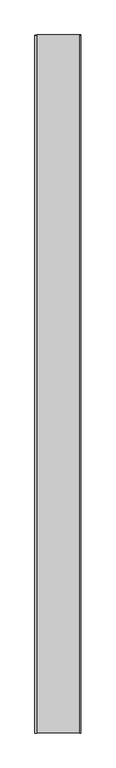
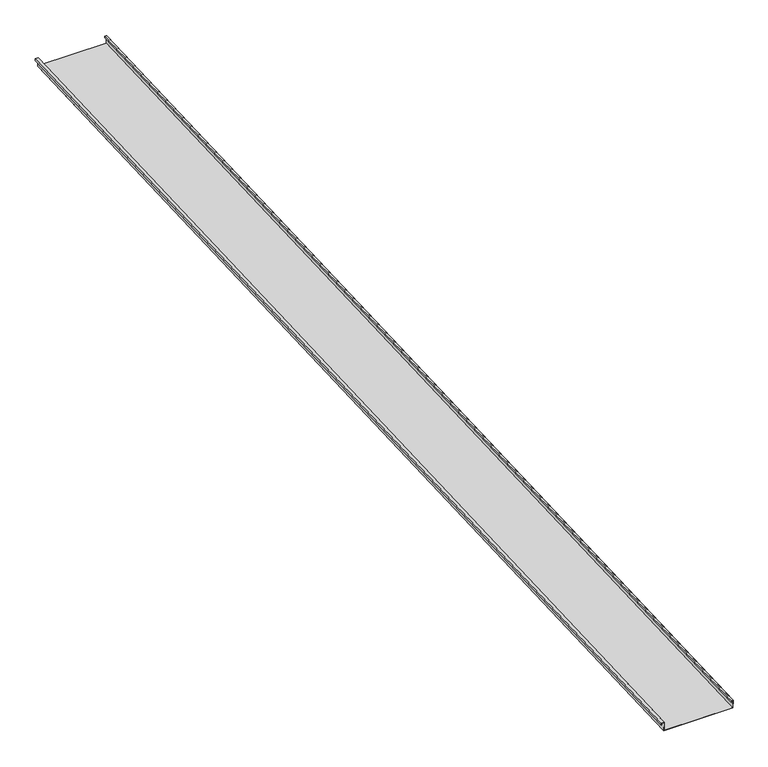
"""IFC4 building model written with IfcOpenShell, lengths in millimetres: proxy geometry, Generic Models 2:Generic Models 2:310765:Generic Models 2:310765 : Generic Models 2:Generic Models 2:310765:112 : Generic Models 2:Generic Models 2:310765:Generic Models 2:310765 : Generic Models 2:Generic Models 2:310765:300385."""

from ifc_helpers import new_model, si_unit, frame, origin, place, context, project, spatial, polyline, outline, extrude, source, transform, mapped, element, save


def generic_models_0e6c4cea(model_context):
    return source(origin(), model_context, "Body", "SweptSolid", [
        extrude(outline(polyline([(1.5875, 0.0), (1.5875, 50.8), (407.9875, 50.8), (407.9875, 1.5875), (396.875, 1.5875), (396.875, 11.1125), (398.4625, 11.1125), (398.4625, 3.175), (406.4, 3.175), (406.4, 49.2125), (3.175, 49.2125), (3.175, -1.5874999), (-14.2875, -1.5874999), (-14.2875, 9.525), (-12.7, 9.525), (-12.7, 0.0), (1.5875, 0.0)])), frame((608242.8096406, -581354.4345603, 3902.6697972), z_axis=(0.0, 0.9991330730923568, 0.041630544712067834), x_axis=(1.0, 0.0, 0.0)), (0.0, 0.0, 1.0), 6400.8),
    ])


if __name__ == "__main__":
    model = new_model("IFC4")
    model_context = context("Model", 3, world=origin())
    ifc_project = project(units=[si_unit("LENGTHUNIT", "METRE", prefix="MILLI")], contexts=[model_context])
    site = spatial("IfcSite", under=ifc_project)
    building = spatial("IfcBuilding", under=site)
    placement = place(None, origin())
    generic_models_shape = generic_models_0e6c4cea(model_context)
    element("IfcBuildingElementProxy", 1, Name="Generic Models 2:Generic Models 2:310765:Generic Models 2:310765 : Generic Models 2:Generic Models 2:310765:112 : Generic Models 2:Generic Models 2:310765:Generic Models 2:310765 : Generic Models 2:Generic Models 2:310765:300385", ObjectType="Generic Models 2:Generic Models 2:310765:Generic Models 2:310765 : Generic Models 2:Generic Models 2:310765:112 : Generic Models 2:Generic Models 2:310765:Generic Models 2:310765 : Generic Models 2:Generic Models 2:310765:300385", at=placement, inside=building, context=model_context, shape_type="MappedRepresentation", body=[
        mapped(generic_models_shape, transform((0.0, 0.0, 0.0), x_axis=(1.0, 0.0, 0.0), y_axis=(0.0, 1.0, 0.0), z_axis=(0.0, 0.0, 1.0))),
    ])
    save(model, "model.ifc")

# Revit data of these elements
# Type "Generic Models 2:Generic Models 2:310765:Generic Models 2:310765 : Generic Models 2:Generic Models 2:310765:112 : Generic Models 2:Generic Models 2:310765:Generic Models 2:310765 : Generic Models 2:Generic Models 2:310765:300385"
#   NameOverride = "Generic Models 2:Generic Models 2:310765:Generic Models 2:310765 : Generic Models 2:Generic Models 2:310765:300385"
#   ObjectTypeOverride = "Generic Models 2:310765 : Generic Models 2:Generic Models 2:310765"
#   Reference = "Generic Models 2"
#   Tag = "300385"
# Element 1 (IfcBuildingElementProxy, "Generic Models 2:Generic Models 2:310765:Generic Models 2:310765 : Generic Models 2:Generic Models 2:310765:112 : Generic Models 2:Generic Models 2:310765:Generic Models 2:310765 : Generic Models 2:Generic Models 2:310765:300385")
#   Materials on its faces: "THERMAL BROKEN ALUMINUM STOREFRONT FOR POLYCARBONATE"
# Materials
#   "THERMAL BROKEN ALUMINUM STOREFRONT FOR POLYCARBONATE": class "Unassigned", colour RGB 244 244 244, transparency 0, Keynote = "M07611300.01", Cost = 0
